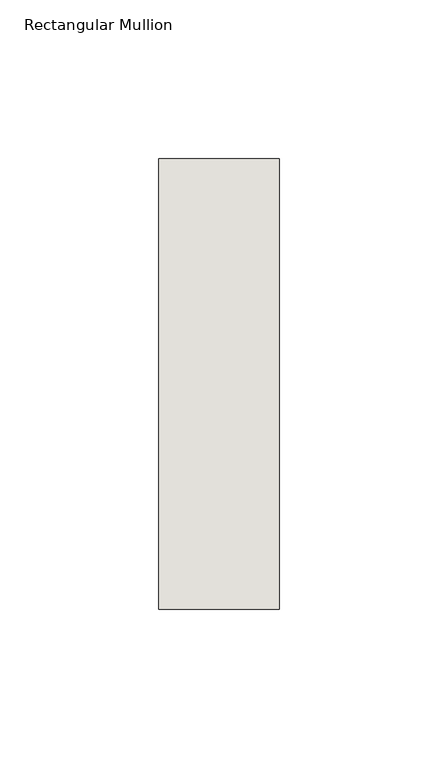
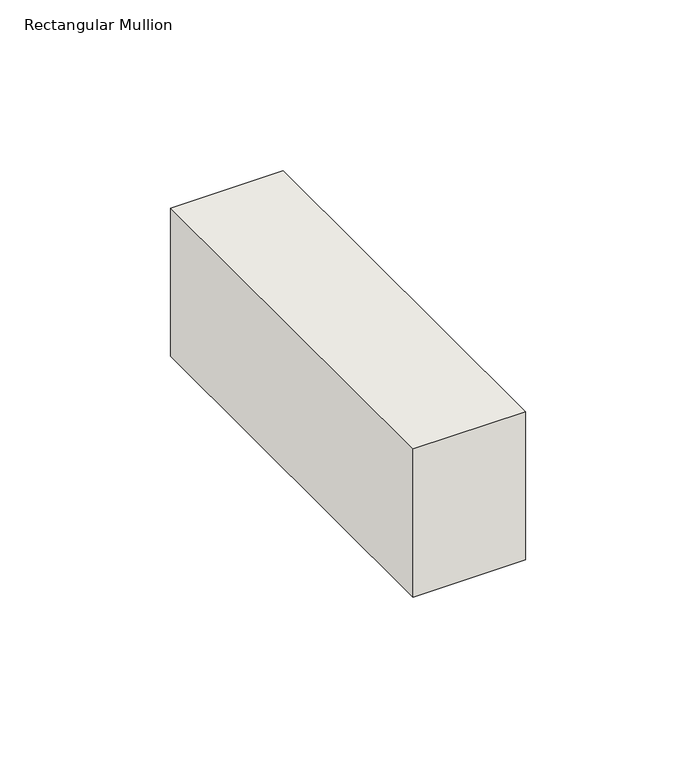
"""IFC4 building model written with IfcOpenShell, lengths in millimetres: wall geometry, Rectangular Mullion : NLRS_21_CWM_hsb-regel 38x142_gen_rsf."""

from ifc_helpers import new_model, si_unit, frame, origin, place, context, project, spatial, polyline, outline, extrude, source, transform, mapped, element, save


def rectangular_mullion_7080d8a8(model_context):
    return source(origin(), model_context, "Body", "SweptSolid", [
        extrude(outline(polyline([(-38.0, -71.0), (-38.0, 71.0), (0.0, 71.0), (0.0, -71.0), (-38.0, -71.0)])), frame((0.0, 0.0, -52.9999997), z_axis=(0.0, 0.0, 1.0), x_axis=(1.0, 0.0, 0.0)), (0.0, 0.0, 1.0), 52.9999997),
    ])


if __name__ == "__main__":
    model = new_model("IFC4")
    model_context = context("Model", 3, world=origin())
    ifc_project = project(units=[si_unit("LENGTHUNIT", "METRE", prefix="MILLI")], contexts=[model_context])
    site = spatial("IfcSite", under=ifc_project)
    building = spatial("IfcBuilding", under=site)
    placement = place(None, origin())
    rectangular_mullion_shape = rectangular_mullion_7080d8a8(model_context)
    element("IfcWall", 1, ObjectType="Rectangular Mullion : NLRS_21_CWM_hsb-regel 38x142_gen_rsf", at=placement, inside=building, context=model_context, shape_type="MappedRepresentation", body=[
        mapped(rectangular_mullion_shape, transform((0.0, 0.0, 0.0), x_axis=(1.0, 0.0, 0.0), y_axis=(0.0, 1.0, 0.0), z_axis=(0.0, 0.0, 1.0))),
    ])
    save(model, "model.ifc")

# Revit data of these elements
# Type "Rectangular Mullion : NLRS_21_CWM_hsb-regel 38x142_gen_rsf"
#   Type IfcGUID = "07M7mRoiH1CR8m_RSKIwpF"
#   Assembly Code = "21.10"
#   IfcExportAs = "IfcWall"
#   built-in parameter 1007322 = 0.465879 (stored number, unit not read)
#   built-in parameter 1007321 = 0.062336 (stored number, unit not read)
#   built-in parameter 1007320 = 0.062336 (stored number, unit not read)
# Element 1 (IfcWall, "Rectangular Mullion : NLRS_21_CWM_hsb-regel 38x142_gen_rsf")
#   Materials on its faces: "NLRS_i2_hout naaldhout vuren_gen_rsf"
# Materials
#   "NLRS_i2_hout naaldhout vuren_gen_rsf": class "I - Hout", colour RGB 234 199 147, transparency 0, Keynote = "i2", Manufacturer = "Revit Standards Foundation", URL = "www.revitstandards.org", Description = "hout vuren", Cost = 0
